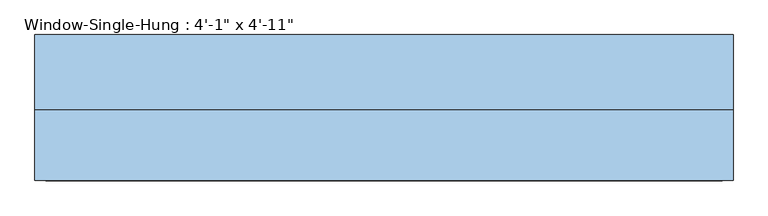
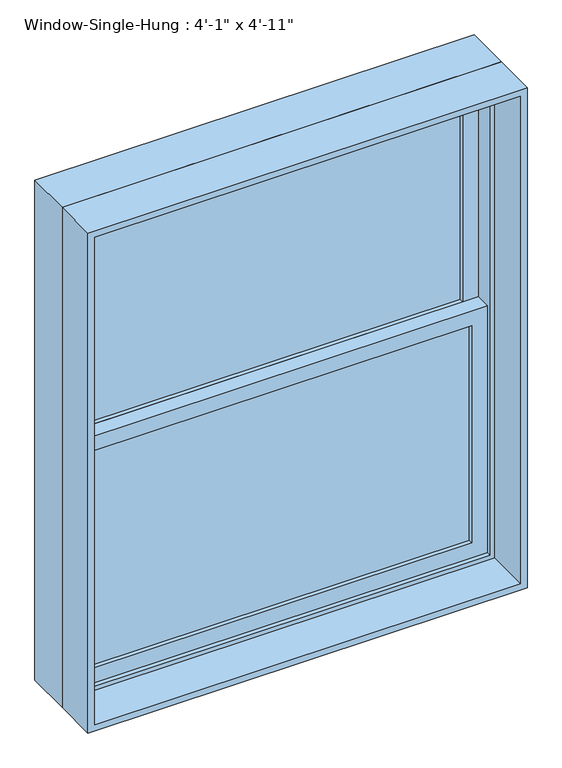
"""IFC4 building model written with IfcOpenShell, lengths in millimetres: window geometry."""

from ifc_helpers import new_model, si_unit, frame, origin, place, context, project, spatial, polyline, outline, extrude, source, transform, mapped, element, save


def window_28033f45(model_context):
    return source(origin(), model_context, "Body", "SweptSolid", [
        extrude(outline(polyline([(546.1, 50.8), (546.1, 44.45), (-546.1, 44.45), (-546.1, 50.8), (546.1, 50.8)])), frame((0.0, 0.0, 990.6), z_axis=(0.0, 0.0, 1.0), x_axis=(1.0, 0.0, 0.0)), (0.0, 0.0, 1.0), 650.875),
        extrude(outline(polyline([(-546.1, 38.1), (546.1, 38.1), (546.1, 31.75), (-546.1, 31.75), (-546.1, 38.1)])), frame((0.0, 0.0, 990.6), z_axis=(0.0, 0.0, 1.0), x_axis=(1.0, 0.0, 0.0)), (0.0, 0.0, 1.0), 650.875),
        extrude(outline(polyline([(546.1, 95.25), (546.1, 88.9), (-546.1, 88.9), (-546.1, 95.25), (546.1, 95.25)])), frame((0.0, 0.0, 1685.925), z_axis=(0.0, 0.0, 1.0), x_axis=(1.0, 0.0, 0.0)), (0.0, 0.0, 1.0), 650.875),
        extrude(outline(polyline([(-546.1, 82.55), (546.1, 82.55), (546.1, 76.2), (-546.1, 76.2), (-546.1, 82.55)])), frame((0.0, 0.0, 1685.925), z_axis=(0.0, 0.0, 1.0), x_axis=(1.0, 0.0, 0.0)), (0.0, 0.0, 1.0), 650.875),
        extrude(outline(polyline([(1685.925, -590.55), (946.15, -590.55), (946.15, 590.55), (1685.925, 590.55), (1685.925, -590.55)]), holes=[polyline([(1641.475, 546.1), (990.6, 546.1), (990.6, -546.1), (1641.475, -546.1), (1641.475, 546.1)])]), frame((0.0, 19.05, 0.0), z_axis=(0.0, 1.0, 0.0), x_axis=(0.0, 0.0, 1.0)), (0.0, 0.0, 1.0), 44.45),
        extrude(outline(polyline([(2381.25, -590.55), (1641.475, -590.55), (1641.475, 590.55), (2381.25, 590.55), (2381.25, -590.55)]), holes=[polyline([(2336.8, 546.1), (1685.925, 546.1), (1685.925, -546.1), (2336.8, -546.1), (2336.8, 546.1)])]), frame((0.0, 63.5, 0.0), z_axis=(0.0, 1.0, 0.0), x_axis=(0.0, 0.0, 1.0)), (0.0, 0.0, 1.0), 44.45),
        extrude(outline(polyline([(2413.0, -622.3), (914.4, -622.3), (914.4, 622.3), (2413.0, 622.3), (2413.0, -622.3)]), holes=[polyline([(2381.25, 590.55), (946.15, 590.55), (946.15, -590.55), (2381.25, -590.55), (2381.25, 590.55)])]), frame((0.0, 6.35, 0.0), z_axis=(0.0, 1.0, 0.0), x_axis=(0.0, 0.0, 1.0)), (0.0, 0.0, 1.0), 133.35),
        extrude(outline(polyline([(2413.0, 622.3), (2413.0, -622.3), (914.4, -622.3), (914.4, 622.3), (2413.0, 622.3)]), holes=[polyline([(2393.95, 603.25), (933.45, 603.25), (933.45, -603.25), (2393.95, -603.25), (2393.95, 603.25)])]), frame((0.0, -120.65, 0.0), z_axis=(0.0, 1.0, 0.0), x_axis=(0.0, 0.0, 1.0)), (0.0, 0.0, 1.0), 127.0),
    ])


if __name__ == "__main__":
    model = new_model("IFC4")
    model_context = context("Model", 3, world=origin())
    ifc_project = project(units=[si_unit("LENGTHUNIT", "METRE", prefix="MILLI")], contexts=[model_context])
    site = spatial("IfcSite", under=ifc_project)
    building = spatial("IfcBuilding", under=site)
    placement = place(None, origin())
    window_shape = window_28033f45(model_context)
    element("IfcWindow", 1, ObjectType="Window-Single-Hung : 4'-1\" x 4'-11\"", at=placement, inside=building, context=model_context, shape_type="MappedRepresentation", body=[
        mapped(window_shape, transform((0.0, 0.0, 0.0), x_axis=(1.0, 0.0, 0.0), y_axis=(0.0, 1.0, 0.0), z_axis=(0.0, 0.0, 1.0))),
    ])
    save(model, "model.ifc")

# Revit data of these elements
# Type "Window-Single-Hung : 4'-1\" x 4'-11\""
#   Type Mark = "02"
#   Fire Rating = "0.5h"
#   Construction Type Id = "DG-DR"
#   Assembly Code = "B2020100"
#   Analytic Construction = "Double glazing - domestic"
#   Wall Thickness [instance default] = 0' - 6"
#   Window Inset [instance default] = 0' - 0"
#   Visual Light Transmittance = 0.81
#   Thermal Resistance (R) = 0.319569 (m²·K)/W
#   Solar Heat Gain Coefficient = 0.76
#   Muntin Width = 3' - 7"
#   Muntin Height = 2' - 1 5/8"
#   Interior Wall Closure [instance default] = 0' - 1 1/2"
#   Rough Width = 4' - 1 1/2"
#   Rough Height = 4' - 11 1/2"
#   Frame Extension [instance default] = 0' - 1 1/4"
#   Exterior Wall Closure [instance default] = 0' - 0 1/2"
#   Extension Jamb [instance default] = 0' - 1 1/2"
#   Heat Transfer Coefficient (U) = 3.12929 W/(m²·K)
#   Height = 4' - 11"
#   Width = 4' - 1"
#   Top Muntin Visibility = no
#   Indicator Visibility = no
#   Extension Jamb Visibility [instance default] = yes
#   Interior Trim Visibility [instance default] = yes
#   Exterior Trim Visibility [instance default] = yes
#   Bottom Muntin Visibility = no
#   Muntin Pattern = Muntin Pattern_2x2 : Muntin Pattern_2x2
#   Interior Trim Material = 1X WOOD COMPOSITE TRIM
#   Interior Trim = Trim-Window-Interior-Flat : Picture Frame
#   Exterior Trim Material = 1X WOOD COMPOSITE TRIM
#   Exterior Trim = Trim-Window-Exterior-Flat : with Sill
#   Glass Panel Material = NEW DOUBLE HUNG WINDOWS (TYP.)
#   Exterior Frame Material = 1X WOOD COMPOSITE TRIM
#   Interior Frame Material = 1X WOOD COMPOSITE TRIM
#   Wall Closure = (empty or 0)
# Element 1 (IfcWindow, "Window-Single-Hung : 4'-1\" x 4'-11\"")
#   Wall Thickness = 0' - 9 1/2"
#   Extension Jamb = 0' - 5"
#   Materials on its faces: "1X WOOD COMPOSITE TRIM", "NEW DOUBLE HUNG WINDOWS (TYP.)"
# Materials
#   "1X WOOD COMPOSITE TRIM": class "Generic", colour RGB 88 61 61, transparency 0, Cost = 0
#   "NEW DOUBLE HUNG WINDOWS (TYP.)": class "Glass", colour RGB 218 227 224, transparency 0.85, Description = "Soda Lime Glass", Cost = 0
